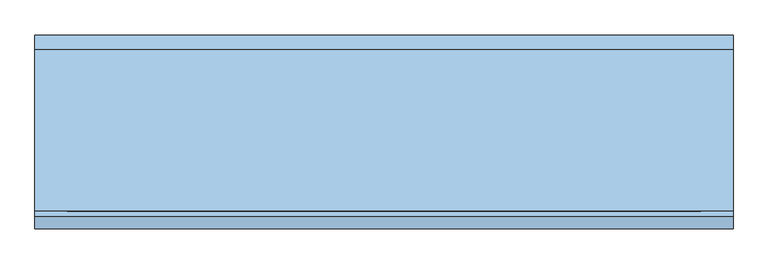
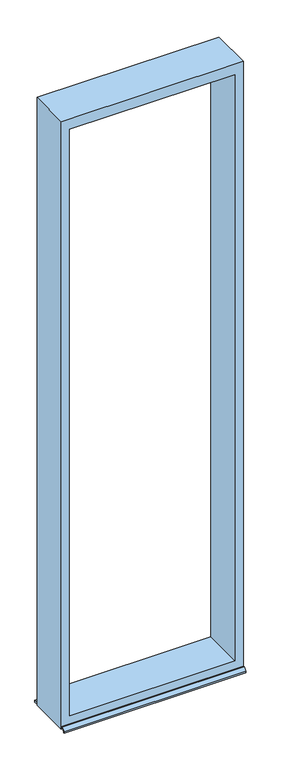
"""IFC4 building model written with IfcOpenShell, lengths in millimetres: window geometry, Fenster - Festverglasung : Feste Verglasung 4.58 x 1.31 3 2."""

from ifc_helpers import new_model, si_unit, frame, origin, place, context, project, spatial, polyline, outline, extrude, source, transform, mapped, element, save


def window_884f6abb(model_context):
    return source(origin(), model_context, "Body", "SweptSolid", [
        extrude(outline(polyline([(5580.0, 650.0), (5580.0, -650.0), (1000.0, -650.0), (1000.0, 650.0), (5580.0, 650.0)]), holes=[polyline([(5500.0, 590.0), (1080.0, 590.0), (1080.0, -590.0), (5500.0, -590.0), (5500.0, 590.0)])]), frame((0.0, -147.5214598, 0.0), z_axis=(0.0, 1.0, 0.0), x_axis=(0.0, 0.0, 1.0)), (0.0, 0.0, 1.0), 300.0),
        extrude(outline(polyline([(-650.0, 180.0), (650.0, 180.0), (650.0, 152.4785402), (-650.0, 152.4785402), (-650.0, 180.0)])), frame((0.0, 0.0, 1005.0), z_axis=(0.0, 0.0, 1.0), x_axis=(1.0, 0.0, 0.0)), (0.0, 0.0, 1.0), 15.0),
        extrude(outline(polyline([(-157.5436142, 1020.0), (-147.5214598, 1020.0), (-147.5214598, 1018.0), (-157.3455321, 1018.0), (-178.0, 998.3604634), (-178.0, 990.0), (-180.0, 990.0), (-180.0, 1000.0), (-157.5436142, 1020.0)])), frame((-650.0, 0.0, 0.0), z_axis=(1.0, 0.0, 0.0), x_axis=(0.0, 1.0, 0.0)), (0.0, 0.0, 1.0), 1300.0),
    ])


if __name__ == "__main__":
    model = new_model("IFC4")
    model_context = context("Model", 3, world=origin())
    ifc_project = project(units=[si_unit("LENGTHUNIT", "METRE", prefix="MILLI")], contexts=[model_context])
    site = spatial("IfcSite", under=ifc_project)
    building = spatial("IfcBuilding", under=site)
    placement = place(None, origin())
    window_shape = window_884f6abb(model_context)
    element("IfcWindow", 1, ObjectType="Fenster - Festverglasung : Feste Verglasung 4.58 x 1.31 3 2", at=placement, inside=building, context=model_context, shape_type="MappedRepresentation", body=[
        mapped(window_shape, transform((0.0, 0.0, 0.0), x_axis=(1.0, 0.0, 0.0), y_axis=(0.0, 1.0, 0.0), z_axis=(0.0, 0.0, 1.0))),
    ])
    save(model, "model.ifc")

# Revit data of these elements
# Type "Fenster - Festverglasung : Feste Verglasung 4.58 x 1.31 3 2"
#   Type Mark = "62"
#   Operation = "SinglePanel"
#   Keynote = "16.05.01"
#   Visual Light Transmittance = 0.9
#   Solar Heat Gain Coefficient = 0.78
#   Rough Width = 1.300 m
#   Rough Height = 4.580 m
#   Heat Transfer Coefficient (U) = 3.6886 W/(m²·K)
#   Rahmentiefe = 0.300 m
#   Rahmenhöhe unten = 0.080 m
#   Höhe oberer  Rahmen = 0.080 m
#   Rahmenbreite = 0.060 m
#   Height = 4.580 m
#   Einbautiefe (von außen) [instance default] = 0.080 m
#   Width = 1.300 m
#   Wall Closure = 3
#   Bild [instance default] = none
#   Glas [instance default] = none
#   Innere Fensterbank [instance default] = none
#   Äußere Fensterbank [instance default] = none
#   Construction Type Id = ""
#   Analytic Construction = (empty or 0)
# Element 1 (IfcWindow, "Fenster - Festverglasung : Feste Verglasung 4.58 x 1.31 3 2")
#   Einbautiefe (von außen) = 0.002479 m
#   Materials on its faces: "Kunststoff - Weiß", "Holz - Birke"
# Materials
#   "Kunststoff - Weiß": class "Kunststoff", colour RGB 249 249 249, transparency 0, Cost = 0
#   "Holz - Birke": class "Holz", colour RGB 213 164 103, transparency 0, Cost = 0
